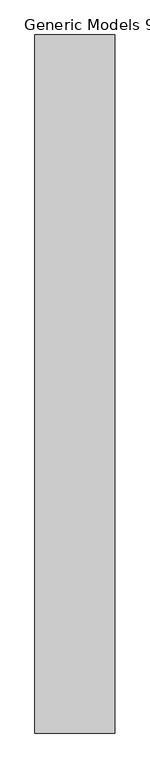
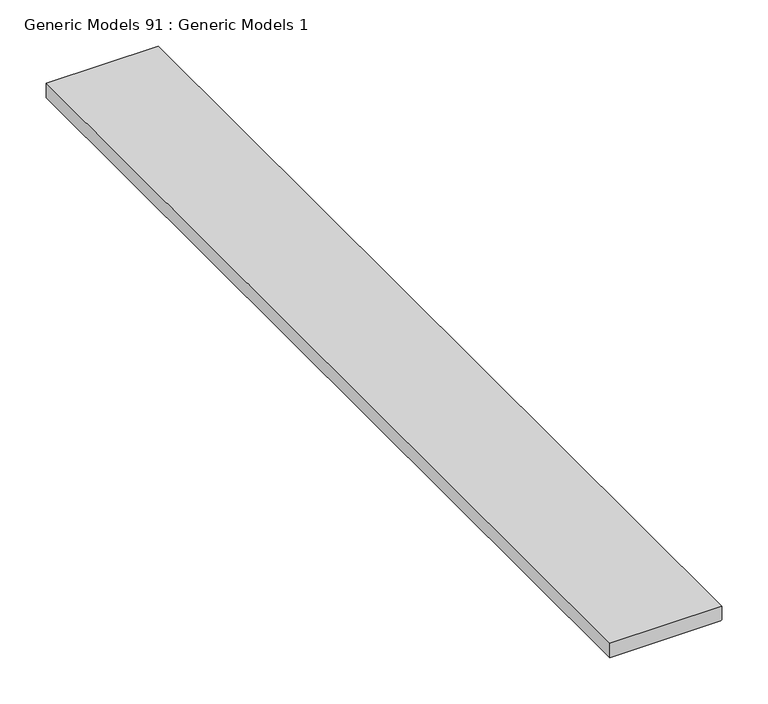
"""IFC4 building model written with IfcOpenShell, lengths in millimetres: proxy geometry, Generic Models 91 : Generic Models 1."""

import ifcopenshell
import ifcopenshell.guid

model = None  # the IFC model being written
_history = None  # IfcOwnerHistory: only IFC2X3 demands one
_inside = {}  # id of a spatial element -> (the spatial element, [elements in it])
_under = {}  # id of a project, library or spatial element -> (it, [spatial elements below it])
_declared = {}  # id of a project -> (the project, [libraries it declares])
_typed = {}  # id of a type object -> (the type object, [elements of that type])
_made_of = {}  # id of a material, layer set ... -> (it, [elements and type objects made of it])


def new_model(schema):
    """Start an empty IFC model of exactly this schema.

    Asked for "IFC4X3", IfcOpenShell would pick the latest addendum, in which some entities
    have other attributes; the version numbers below select the first issue.
    IFC2X3 requires an IfcOwnerHistory on every rooted entity: one is made here for all.
    """
    global model, _history
    if schema == "IFC4X3":
        model = ifcopenshell.file(schema_version=(4, 3, 0, 0))
    else:
        model = ifcopenshell.file(schema=schema)
    _inside.clear()
    _under.clear()
    _declared.clear()
    _typed.clear()
    _made_of.clear()
    _history = None
    if model.schema == "IFC2X3":
        org = make("IfcOrganization", Name="unknown")
        user = make(
            "IfcPersonAndOrganization",
            ThePerson=make("IfcPerson", FamilyName="unknown"),
            TheOrganization=org,
        )
        app = make(
            "IfcApplication",
            ApplicationDeveloper=org,
            Version="unknown",
            ApplicationFullName="unknown",
            ApplicationIdentifier="unknown",
        )
        _history = make(
            "IfcOwnerHistory",
            OwningUser=user,
            OwningApplication=app,
            ChangeAction="ADDED",
            CreationDate=0,
        )
    return model


def make(cls, **values):
    """One entity of the class cls with the attributes given. An attribute that is None is left unset."""
    return model.create_entity(
        cls, **{name: value for name, value in values.items() if value is not None}
    )


def rooted(cls, **values):
    """An entity with a GlobalId (a new one), such as an element, a storey or a relation."""
    return make(cls, GlobalId=ifcopenshell.guid.new(), OwnerHistory=_history, **values)


def si_unit(unit_type, name, prefix=None):
    """IfcSIUnit, for example si_unit("LENGTHUNIT", "METRE", prefix="MILLI")."""
    return make("IfcSIUnit", UnitType=unit_type, Prefix=prefix, Name=name)


def assignment(units):
    """IfcUnitAssignment: the units of a project."""
    return None if units is None else make("IfcUnitAssignment", Units=units)


def point(xyz):
    """IfcCartesianPoint."""
    return None if xyz is None else make("IfcCartesianPoint", Coordinates=xyz)


def direction(xyz):
    """IfcDirection."""
    return None if xyz is None else make("IfcDirection", DirectionRatios=xyz)


def frame(location, z_axis=None, x_axis=None):
    """IfcAxis2Placement3D, a coordinate frame: its origin and axes. An axis left out is left unset."""
    return make(
        "IfcAxis2Placement3D",
        Location=point(location),
        Axis=direction(z_axis),
        RefDirection=direction(x_axis),
    )


def origin():
    """The frame at (0, 0, 0) with its axes left unset."""
    return frame((0.0, 0.0, 0.0))


def place(relative_to, where):
    """IfcLocalPlacement: puts the frame where relative to a parent placement (None: the world)."""
    return make(
        "IfcLocalPlacement", PlacementRelTo=relative_to, RelativePlacement=where
    )


def context(
    kind, dimensions, precision=None, world=None, true_north=None, identifier=None
):
    """IfcGeometricRepresentationContext, for example the 3D "Model" context."""
    return make(
        "IfcGeometricRepresentationContext",
        ContextIdentifier=identifier,
        ContextType=kind,
        CoordinateSpaceDimension=dimensions,
        Precision=precision,
        WorldCoordinateSystem=world,
        TrueNorth=true_north,
    )


def project(units=None, contexts=None):
    """IfcProject with its units and contexts."""
    return rooted(
        "IfcProject",
        Name="project",
        RepresentationContexts=contexts,
        UnitsInContext=assignment(units),
    )


def spatial(cls, under=None, at=None, **own):
    """A site, building, storey or space (cls), placed at a placement, below another one or the project."""
    s = rooted(cls, ObjectPlacement=at, **own)
    if under is not None:
        _under.setdefault(under.id(), (under, []))[1].append(s)
    return s


def polyline(points):
    """IfcPolyline through the points."""
    return make("IfcPolyline", Points=[point(p) for p in points])


def outline(outer, holes=None, kind="AREA"):
    """IfcArbitraryClosedProfileDef: a profile drawn as a closed curve; with holes, ...WithVoids."""
    if holes is None:
        return make("IfcArbitraryClosedProfileDef", ProfileType=kind, OuterCurve=outer)
    return make(
        "IfcArbitraryProfileDefWithVoids",
        ProfileType=kind,
        OuterCurve=outer,
        InnerCurves=holes,
    )


def extrude(swept, where, along, depth):
    """IfcExtrudedAreaSolid: the profile swept, set in the frame where, extruded along a direction by depth."""
    return make(
        "IfcExtrudedAreaSolid",
        SweptArea=swept,
        Position=where,
        ExtrudedDirection=direction(along),
        Depth=depth,
    )


def shape(context_of_items, identifier, shape_type, items):
    """IfcShapeRepresentation: the items that make up one representation, for example the "Body"."""
    return make(
        "IfcShapeRepresentation",
        ContextOfItems=context_of_items,
        RepresentationIdentifier=identifier,
        RepresentationType=shape_type,
        Items=items,
    )


def source(mapping_origin, context_of_items, identifier, shape_type, items):
    """IfcRepresentationMap: a shape defined once, which mapped items show again and again."""
    return make(
        "IfcRepresentationMap",
        MappingOrigin=mapping_origin,
        MappedRepresentation=shape(context_of_items, identifier, shape_type, items),
    )


def transform(
    local_origin,
    x_axis=None,
    y_axis=None,
    z_axis=None,
    scale=None,
    scale2=None,
    scale3=None,
    uniform=True,
):
    """IfcCartesianTransformationOperator3D, or its non-uniform kind. x_axis, y_axis, z_axis: its Axis1, 2, 3."""
    if uniform:
        return make(
            "IfcCartesianTransformationOperator3D",
            Axis1=direction(x_axis),
            Axis2=direction(y_axis),
            LocalOrigin=point(local_origin),
            Scale=scale,
            Axis3=direction(z_axis),
        )
    return make(
        "IfcCartesianTransformationOperator3DnonUniform",
        Axis1=direction(x_axis),
        Axis2=direction(y_axis),
        LocalOrigin=point(local_origin),
        Scale=scale,
        Axis3=direction(z_axis),
        Scale2=scale2,
        Scale3=scale3,
    )


def mapped(mapping_source, mapping_target):
    """IfcMappedItem: shows the shape of a source again, moved by a transform."""
    return make(
        "IfcMappedItem", MappingSource=mapping_source, MappingTarget=mapping_target
    )


def made_of(thing, what):
    """Note that an element or type object is made of a material, layer set ...; save() writes the relation."""
    if what is not None:
        _made_of.setdefault(what.id(), (what, []))[1].append(thing)
    return thing


def element(
    cls,
    number,
    at=None,
    inside=None,
    cuts=None,
    type_object=None,
    material=None,
    context=None,
    identifier="Body",
    shape_type=None,
    held_by="IfcProductDefinitionShape",
    body=None,
    shapes=None,
    **own,
):
    """One element of the class cls, such as IfcWall. Its Tag is "e" and its number.

    at: its placement. inside: the storey or other place that contains it. cuts: it is an
    opening in that element (IfcRelVoidsElement). A single representation is given by context,
    identifier, shape_type and body (its items); several are given by shapes. held_by: the class
    of the entity that holds the representations. save() writes the other relations.
    """
    e = rooted(cls, Tag="e%d" % number, ObjectPlacement=at, **own)
    if body is not None:
        shapes = [shape(context, identifier, shape_type, body)]
    if shapes is not None:
        e.Representation = make(held_by, Representations=shapes)
    if inside is not None:
        _inside.setdefault(inside.id(), (inside, []))[1].append(e)
    if cuts is not None:
        rooted(
            "IfcRelVoidsElement", RelatingBuildingElement=cuts, RelatedOpeningElement=e
        )
    if type_object is not None:
        _typed.setdefault(type_object.id(), (type_object, []))[1].append(e)
    return made_of(e, material)


def aggregate(whole, parts):
    """IfcRelAggregates: a whole, such as a stair, and the parts it consists of."""
    return rooted("IfcRelAggregates", RelatingObject=whole, RelatedObjects=parts)


def save(model, path):
    """Write the relations noted so far, then the file.

    IfcRelAggregates (storeys below a building ...), IfcRelContainedInSpatialStructure (elements
    in a storey), IfcRelDefinesByType, IfcRelAssociatesMaterial and IfcRelDeclares: one each for
    every whole, place, type object, material and project.
    """
    for whole, parts in _under.values():
        aggregate(whole, parts)
    for where, things in _inside.values():
        rooted(
            "IfcRelContainedInSpatialStructure",
            RelatedElements=things,
            RelatingStructure=where,
        )
    for kind, things in _typed.values():
        rooted("IfcRelDefinesByType", RelatedObjects=things, RelatingType=kind)
    for what, things in _made_of.values():
        rooted("IfcRelAssociatesMaterial", RelatedObjects=things, RelatingMaterial=what)
    for by, libraries in _declared.values():
        rooted("IfcRelDeclares", RelatingContext=by, RelatedDefinitions=libraries)
    model.write(path)


def generic_models_91_generic_models_1_98bef9af(model_context):
    return source(origin(), model_context, "Body", "SweptSolid", [
        extrude(outline(polyline([(2250.523933, 45484.8985531), (2250.523933, 45623.4079281), (2251.714558, 45624.5985531), (2269.573933, 45624.5985531), (2269.573933, 45484.8985531), (2250.523933, 45484.8985531)])), frame((0.0, 0.0, 0.0), z_axis=(0.0, 1.0, 0.0), x_axis=(0.0, 0.0, 1.0)), (0.0, 0.0, 1.0), 1219.2),
    ])


if __name__ == "__main__":
    model = new_model("IFC4")
    model_context = context("Model", 3, world=origin())
    ifc_project = project(units=[si_unit("LENGTHUNIT", "METRE", prefix="MILLI")], contexts=[model_context])
    site = spatial("IfcSite", under=ifc_project)
    building = spatial("IfcBuilding", under=site)
    placement = place(None, origin())
    generic_models_91_generic_models_1_shape = generic_models_91_generic_models_1_98bef9af(model_context)
    element("IfcBuildingElementProxy", 1, Name="Generic Models 91 : Generic Models 1", ObjectType="Generic Models 91 : Generic Models 1", at=placement, inside=building, context=model_context, shape_type="MappedRepresentation", body=[
        mapped(generic_models_91_generic_models_1_shape, transform((0.0, 0.0, 0.0), x_axis=(1.0, 0.0, 0.0), y_axis=(0.0, 1.0, 0.0), z_axis=(0.0, 0.0, 1.0))),
    ])
    save(model, "model.ifc")

# Revit data of these elements
# Element 1 (IfcBuildingElementProxy, "Generic Models 91 : Generic Models 1")
#   Materials on its faces: "STAINED WOOD TRIM TO MATCH EXISTING"
# Materials
#   "STAINED WOOD TRIM TO MATCH EXISTING": class "Wood", colour RGB 144 113 62, transparency 0, Description = "Pinus Echinata", Cost = 0
